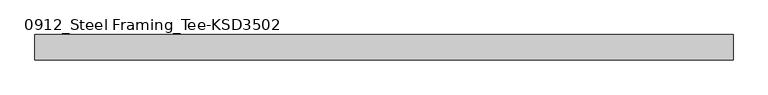
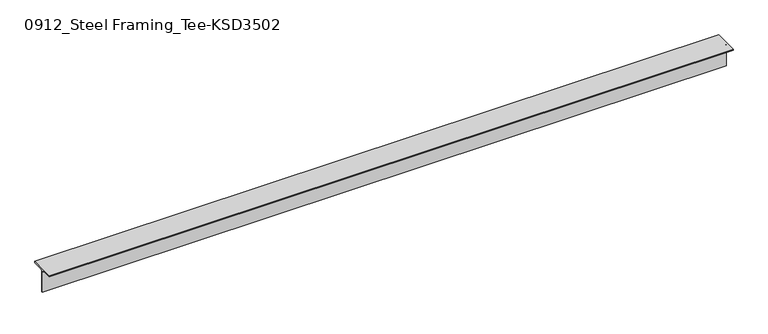
"""IFC4 building model written with IfcOpenShell, lengths in millimetres: member geometry, 0912_Steel Framing_Tee-KSD3502 : H_SB_ASB_CT-150x150x6.5x9."""

from ifc_helpers import new_model, si_unit, point, frame, frame_2d, origin, place, context, project, spatial, polyline, circle_curve, trimmed, segment, composite_curve, outline, extrude, source, transform, mapped, element, save


def member_0912_steel_framing_tee_ksd3502_aad18543(model_context):
    return source(origin(), model_context, "Body", "SweptSolid", [
        extrude(outline(composite_curve([segment(polyline([(-75.0, 75.0), (75.0, 75.0), (75.0, 66.0), (16.25, 66.0)]), True, "CONTINUOUS"), segment(trimmed(circle_curve(frame_2d((16.25, 53.0)), 13.0), [point((16.25, 66.0))], [point((3.25, 53.0))], True, "CARTESIAN"), True, "CONTINUOUS"), segment(polyline([(3.25, 53.0), (3.25, -75.0), (-3.25, -75.0), (-3.25, 53.0)]), True, "CONTINUOUS"), segment(trimmed(circle_curve(frame_2d((-16.25, 53.0)), 13.0), [point((-3.25, 53.0))], [point((-16.25, 66.0))], True, "CARTESIAN"), True, "CONTINUOUS"), segment(polyline([(-16.25, 66.0), (-75.0, 66.0), (-75.0, 75.0)]), True, "CONTINUOUS")], self_intersect=False)), frame((-2106.2, 0.0, 0.0), z_axis=(1.0, 0.0, 0.0), x_axis=(0.0, 1.0, 0.0)), (0.0, 0.0, 1.0), 4152.3),
    ])


if __name__ == "__main__":
    model = new_model("IFC4")
    model_context = context("Model", 3, world=origin())
    ifc_project = project(units=[si_unit("LENGTHUNIT", "METRE", prefix="MILLI")], contexts=[model_context])
    site = spatial("IfcSite", under=ifc_project)
    building = spatial("IfcBuilding", under=site)
    placement = place(None, origin())
    member_0912_steel_framing_tee_ksd3502_shape = member_0912_steel_framing_tee_ksd3502_aad18543(model_context)
    element("IfcMember", 1, ObjectType="0912_Steel Framing_Tee-KSD3502 : H_SB_ASB_CT-150x150x6.5x9", at=placement, inside=building, context=model_context, shape_type="MappedRepresentation", body=[
        mapped(member_0912_steel_framing_tee_ksd3502_shape, transform((0.0, 0.0, 0.0), x_axis=(1.0, 0.0, 0.0), y_axis=(0.0, 1.0, 0.0), z_axis=(0.0, 0.0, 1.0))),
    ])
    save(model, "model.ifc")

# Revit data of these elements
# Type "0912_Steel Framing_Tee-KSD3502 : H_SB_ASB_CT-150x150x6.5x9"
#   H_WM Code_1 = "S01AA003-00001 | Main Steel Structure Fabrication Work | Shelter/Building | Light Steel - Standard (30KG/M>Weight) | Material: (   )"
#   H_WM Code_2 = "S03AA029-00001 | Main Steel Structure Erection Work | Shelter/Building | Light Steel (30KG/M>Weight) | Material: (   )"
#   H_WM Code_3 = "S01AA010-00001 | Main Steel Structure Fabrication Work | Shelter/Building | Steel Painting/Coating | for Non-Fireproofed Steel Surface, Surface Preparation, Primer, Second & Final Coat | Material: (   )"
#   H_Q'ty Cal Type Tag = "SB-Q2"
#   Width = 15.0 cm
#   Web Thickness = 0.65 cm
#   Web Fillet = 1.3 cm
#   Section Area = 23.39 cm²
#   Perimeter = 0.60 m²/m
#   Nominal Weight = 18.40 kgf/m
#   Height = 15.0 cm
#   Flange Thickness = 0.9 cm
#   Centroid Vertical = 7.5 cm
#   Centroid Horizontal = 7.5 cm
#   Length [instance default] = 1.5000 m
#   Structural Material [instance default] = Steel, 45-345
#   Warping Constant = (empty or 0)
#   Torsional Moment of Inertia = 0
#   Section Name Key = ""
#   Plastic Modulus weak axis = 0
#   Plastic Modulus strong axis = 0
#   Moment of Inertia weak axis = 0
#   Moment of Inertia strong axis = 0
#   Elastic Modulus weak axis = 0
#   Elastic Modulus strong axis = 0
#   Bolt Spacing = 0
#   Assembly Code = ""
# Element 1 (IfcMember, "0912_Steel Framing_Tee-KSD3502 : H_SB_ASB_CT-150x150x6.5x9")
#   Structural Material = none
# Materials
#   "Steel, 45-345": class "Metal", colour RGB 189 187 185, transparency 0, Description = "Steel 345 MPa", Cost = 0
